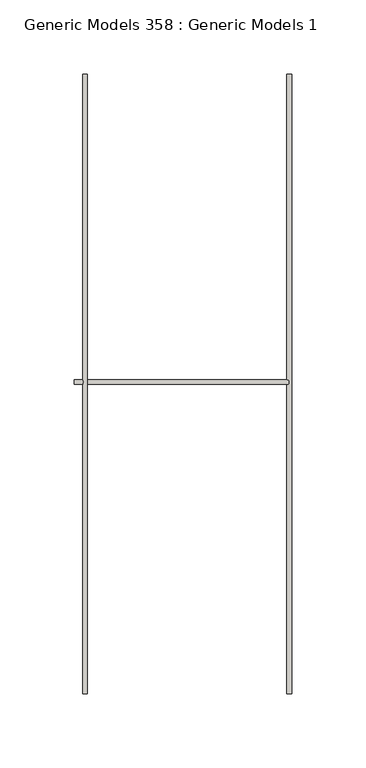
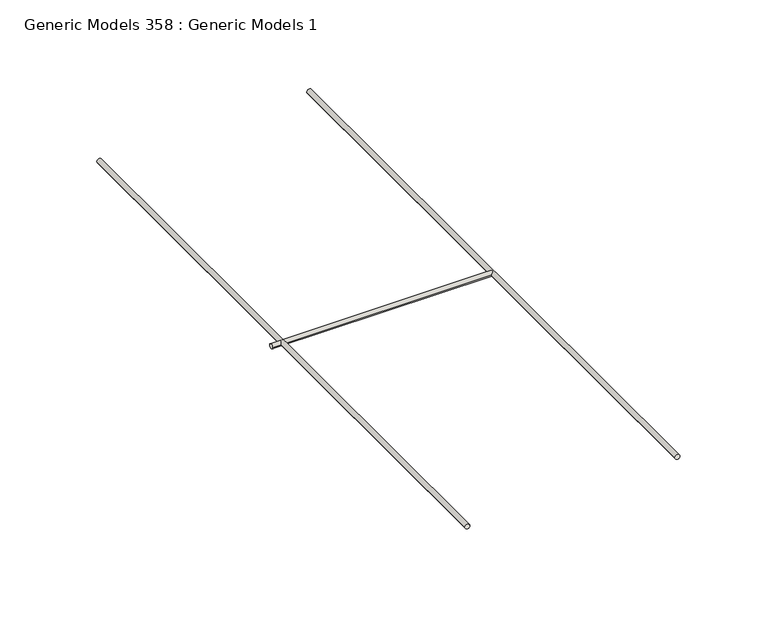
"""IFC4 building model written with IfcOpenShell, lengths in millimetres: wall geometry, Generic Models 358 : Generic Models 1."""

from ifc_helpers import new_model, si_unit, point, frame, frame_2d, origin, place, context, project, spatial, circle_curve, trimmed, segment, composite_curve, outline, extrude, source, transform, mapped, element, save


def generic_models_358_generic_models_1_43605fbf(model_context):
    return source(origin(), model_context, "Body", "SweptSolid", [
        extrude(outline(composite_curve([segment(trimmed(circle_curve(frame_2d((207.8609554, 148397.4894068)), 1.5875), [point((207.8609554, 148399.0769068))], [point((207.8609554, 148395.9019068))], False, "CARTESIAN"), True, "CONTINUOUS"), segment(trimmed(circle_curve(frame_2d((207.8609554, 148397.4894068)), 1.5875), [point((207.8609554, 148395.9019068))], [point((207.8609554, 148399.0769068))], False, "CARTESIAN"), True, "CONTINUOUS")], self_intersect=False)), frame((0.0, 284.6599891, 0.0), z_axis=(0.0, 1.0, 0.0), x_axis=(0.0, 0.0, 1.0)), (0.0, 0.0, 1.0), 417.0150109),
        extrude(outline(composite_curve([segment(trimmed(circle_curve(frame_2d((494.4756823, 207.8609554)), 1.5875), [point((496.0631823, 207.8609554))], [point((492.8881823, 207.8609554))], False, "CARTESIAN"), True, "CONTINUOUS"), segment(trimmed(circle_curve(frame_2d((494.4756823, 207.8609554)), 1.5875), [point((492.8881823, 207.8609554))], [point((496.0631823, 207.8609554))], False, "CARTESIAN"), True, "CONTINUOUS")], self_intersect=False)), frame((148390.2080911, 0.0, 0.0), z_axis=(1.0, 0.0, 0.0), x_axis=(0.0, 1.0, 0.0)), (0.0, 0.0, 1.0), 144.4568621),
        extrude(outline(composite_curve([segment(trimmed(circle_curve(frame_2d((207.8609554, 148534.8605932)), 1.5875), [point((207.8609554, 148533.2730932))], [point((207.8609554, 148536.4480932))], False, "CARTESIAN"), True, "CONTINUOUS"), segment(trimmed(circle_curve(frame_2d((207.8609554, 148534.8605932)), 1.5875), [point((207.8609554, 148536.4480932))], [point((207.8609554, 148533.2730932))], False, "CARTESIAN"), True, "CONTINUOUS")], self_intersect=False)), frame((0.0, 284.6599891, 0.0), z_axis=(0.0, 1.0, 0.0), x_axis=(0.0, 0.0, 1.0)), (0.0, 0.0, 1.0), 417.0150109),
    ])


if __name__ == "__main__":
    model = new_model("IFC4")
    model_context = context("Model", 3, world=origin())
    ifc_project = project(units=[si_unit("LENGTHUNIT", "METRE", prefix="MILLI")], contexts=[model_context])
    site = spatial("IfcSite", under=ifc_project)
    building = spatial("IfcBuilding", under=site)
    placement = place(None, origin())
    generic_models_358_generic_models_1_shape = generic_models_358_generic_models_1_43605fbf(model_context)
    element("IfcWall", 1, ObjectType="Generic Models 358 : Generic Models 1", at=placement, inside=building, context=model_context, shape_type="MappedRepresentation", body=[
        mapped(generic_models_358_generic_models_1_shape, transform((0.0, 0.0, 0.0), x_axis=(1.0, 0.0, 0.0), y_axis=(0.0, 1.0, 0.0), z_axis=(0.0, 0.0, 1.0))),
    ])
    save(model, "model.ifc")

# Revit data of these elements
# Element 1 (IfcWall, "Generic Models 358 : Generic Models 1")
#   Materials on its faces: "STANDARD 9-GAUGE (MW11), LADDER-SHAPED WIRE FABRICATED WITH BUTT-WELDED CROSS-RODS SPACED 406-MM (16-IN.) ON CENTER (OC)"
# Materials
#   "STANDARD 9-GAUGE (MW11), LADDER-SHAPED WIRE FABRICATED WITH BUTT-WELDED CROSS-RODS SPACED 406-MM (16-IN.) ON CENTER (OC)": class "Metal", colour RGB 189 187 185, transparency 0, Description = "Structural steel 50ksi", Cost = 0
